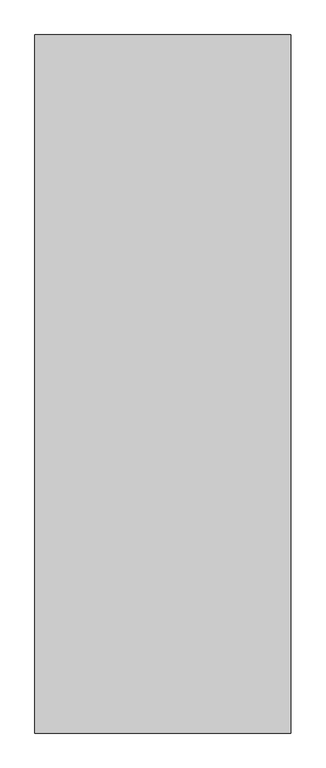
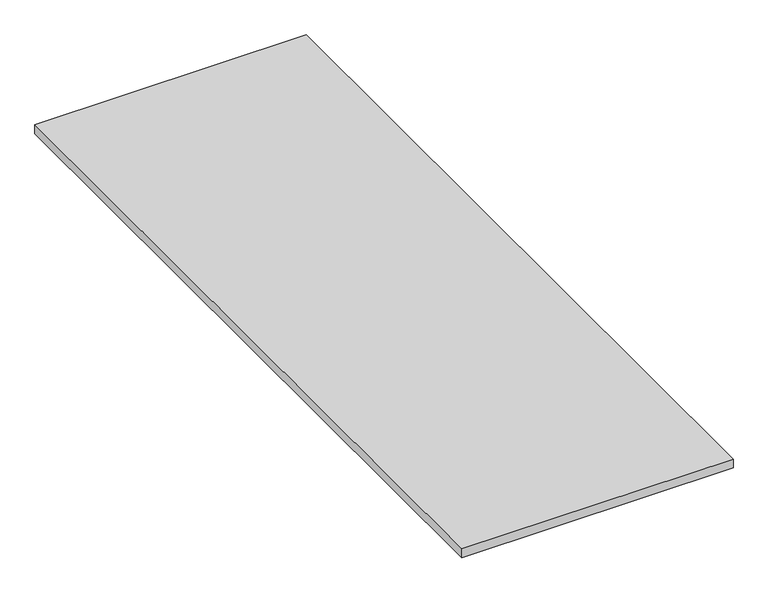
"""IFC4 building model written with IfcOpenShell, lengths in millimetres: proxy geometry, Flooring004 192 : Flooring004 192."""

from ifc_helpers import new_model, si_unit, frame, origin, place, context, project, spatial, polyline, outline, extrude, source, transform, mapped, element, save


def generic_models_689bc37f(model_context):
    return source(origin(), model_context, "Body", "SweptSolid", [
        extrude(outline(polyline([(-8768.1487014, 7982.1529359), (-9501.5737014, 7982.1529359), (-9501.5737014, 9982.1529359), (-8768.1487014, 9982.1529359), (-8768.1487014, 7982.1529359)])), frame((0.0, 0.0, 32594.2960253), z_axis=(0.0, 0.0, 1.0), x_axis=(1.0, 0.0, 0.0)), (0.0, 0.0, 1.0), 25.4),
    ])


if __name__ == "__main__":
    model = new_model("IFC4")
    model_context = context("Model", 3, world=origin())
    ifc_project = project(units=[si_unit("LENGTHUNIT", "METRE", prefix="MILLI")], contexts=[model_context])
    site = spatial("IfcSite", under=ifc_project)
    building = spatial("IfcBuilding", under=site)
    placement = place(None, origin())
    generic_models_shape = generic_models_689bc37f(model_context)
    element("IfcBuildingElementProxy", 1, Name="Flooring004 192 : Flooring004 192", ObjectType="Flooring004 192 : Flooring004 192", at=placement, inside=building, context=model_context, shape_type="MappedRepresentation", body=[
        mapped(generic_models_shape, transform((0.0, 0.0, 0.0), x_axis=(1.0, 0.0, 0.0), y_axis=(0.0, 1.0, 0.0), z_axis=(0.0, 0.0, 1.0))),
    ])
    save(model, "model.ifc")

# Revit data of these elements
# Type "Flooring004 192 : Flooring004 192"
#   NameOverride = "Flooring004"
# Element 1 (IfcBuildingElementProxy, "Flooring004 192 : Flooring004 192")
#   Materials on its faces: "WOOD FLOORING (SPEC TBD)"
# Materials
#   "WOOD FLOORING (SPEC TBD)": class "Unassigned", colour RGB 201 162 125, transparency 0
